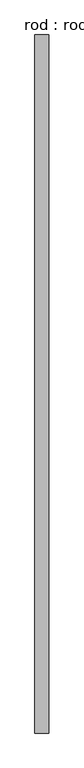
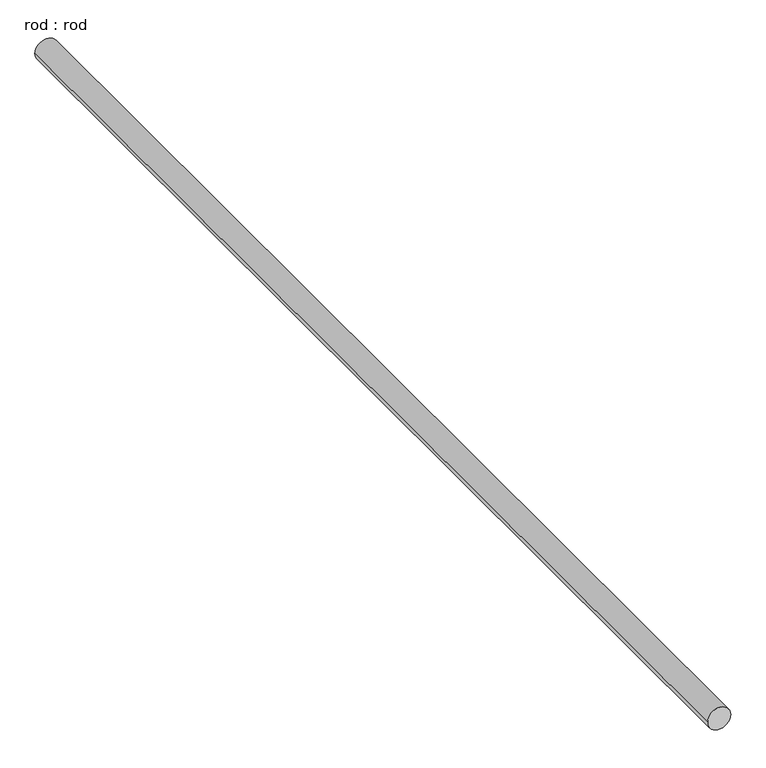
"""IFC4 building model written with IfcOpenShell, lengths in millimetres: proxy geometry, rod : rod."""

from ifc_helpers import new_model, si_unit, point, frame, frame_2d, origin, place, context, project, spatial, circle_curve, trimmed, segment, composite_curve, outline, extrude, source, transform, mapped, element, save


def rod_rod_60a74f7d(model_context):
    return source(origin(), model_context, "Body", "SweptSolid", [
        extrude(outline(composite_curve([segment(trimmed(circle_curve(frame_2d((0.0108462, 0.0)), 200.0), [point((0.0108462, 200.0))], [point((0.0108462, -200.0))], False, "CARTESIAN"), True, "CONTINUOUS"), segment(trimmed(circle_curve(frame_2d((0.0108462, 0.0)), 200.0), [point((0.0108462, -200.0))], [point((0.0108462, 200.0))], False, "CARTESIAN"), True, "CONTINUOUS")], self_intersect=False)), frame((0.0, -6014.4142418, 0.0), z_axis=(0.0, 1.0, 0.0), x_axis=(0.0, 0.0, 1.0)), (0.0, 0.0, 1.0), 20214.2857143),
    ])


if __name__ == "__main__":
    model = new_model("IFC4")
    model_context = context("Model", 3, world=origin())
    ifc_project = project(units=[si_unit("LENGTHUNIT", "METRE", prefix="MILLI")], contexts=[model_context])
    site = spatial("IfcSite", under=ifc_project)
    building = spatial("IfcBuilding", under=site)
    placement = place(None, origin())
    rod_rod_shape = rod_rod_60a74f7d(model_context)
    element("IfcBuildingElementProxy", 1, Name="rod : rod", ObjectType="rod : rod", at=placement, inside=building, context=model_context, shape_type="MappedRepresentation", body=[
        mapped(rod_rod_shape, transform((0.0, 0.0, 0.0), x_axis=(1.0, 0.0, 0.0), y_axis=(0.0, 1.0, 0.0), z_axis=(0.0, 0.0, 1.0))),
    ])
    save(model, "model.ifc")

# Revit data of these elements
# Type "rod : rod"
#   Default Elevation = 0
